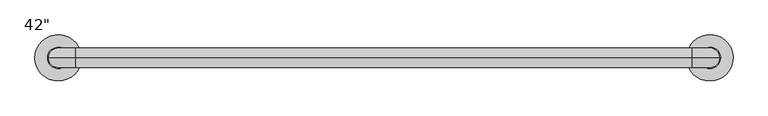
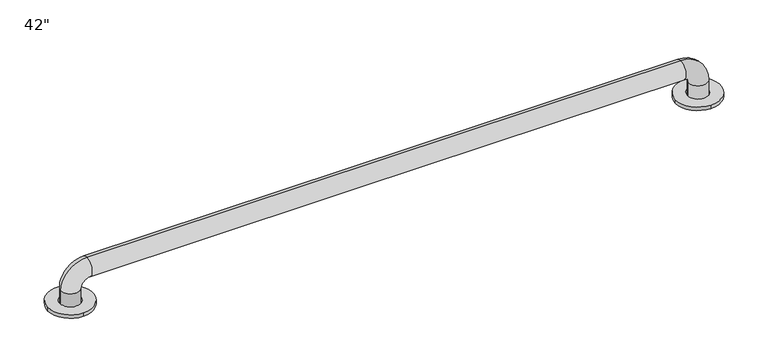
"""IFC4 building model written with IfcOpenShell, lengths in millimetres: proxy geometry."""

from ifc_helpers import new_model, si_unit, point, frame, frame_2d, origin, origin_with_axes, origin_2d, place, context, project, spatial, circle_curve, ellipse_curve, trimmed, segment, composite_curve, outline, extrude, source, transform, mapped, element, save
from ifc_brep_helpers import plane_surface, cylinder_surface, revolved_surface, advanced_brep


def proxy_a4e7295d(model_context):
    return source(origin(), model_context, "Body", "SolidModel", [
        extrude(outline(composite_curve([segment(trimmed(circle_curve(frame_2d((1066.8, 0.0)), 38.1), [point((1028.7, 0.0))], [point((1066.8, -38.1))], False, "CARTESIAN"), True, "CONTINUOUS"), segment(trimmed(circle_curve(frame_2d((1066.8, 0.0)), 38.1), [point((1066.8, -38.1))], [point((1028.7, 0.0))], False, "CARTESIAN"), True, "CONTINUOUS")], self_intersect=False), holes=[composite_curve([segment(trimmed(circle_curve(frame_2d((1066.8, 0.0)), 17.4625), [point((1049.3375, 0.0))], [point((1066.8, -17.4625))], True, "CARTESIAN"), True, "CONTINUOUS"), segment(trimmed(circle_curve(frame_2d((1066.8, 0.0)), 17.4625), [point((1066.8, -17.4625))], [point((1049.3375, 0.0))], True, "CARTESIAN"), True, "CONTINUOUS")], self_intersect=False)]), origin_with_axes(), (0.0, 0.0, 1.0), 6.35),
        extrude(outline(composite_curve([segment(trimmed(circle_curve(origin_2d(), 38.1), [point((-38.1, 0.0))], [point((0.0, -38.1))], False, "CARTESIAN"), True, "CONTINUOUS"), segment(trimmed(circle_curve(origin_2d(), 38.1), [point((0.0, -38.1))], [point((-38.1, 0.0))], False, "CARTESIAN"), True, "CONTINUOUS")], self_intersect=False), holes=[composite_curve([segment(trimmed(circle_curve(origin_2d(), 17.4625), [point((-17.4625, 0.0))], [point((0.0, -17.4625))], True, "CARTESIAN"), True, "CONTINUOUS"), segment(trimmed(circle_curve(origin_2d(), 17.4625), [point((0.0, -17.4625))], [point((-17.4625, 0.0))], True, "CARTESIAN"), True, "CONTINUOUS")], self_intersect=False)]), origin_with_axes(), (0.0, 0.0, 1.0), 6.35),
        advanced_brep(
        [(1082.675, 0.0, 0.0), (1050.925, 0.0, 0.0), (1082.675, 0.0, 28.575), (1050.925, 0.0, 28.575), (1038.225, 0.0, 41.275), (1038.225, 0.0, 73.025), (28.575, 0.0, 73.025), (28.575, 0.0, 41.275), (15.875, 0.0, 28.575), (-15.875, 0.0, 28.575), (-15.875, 0.0, 0.0), (15.875, 0.0, 0.0)],
        [
            (0, 1, circle_curve(frame((1066.8, 0.0, 0.0), z_axis=(0.0, 0.0, -1.0), x_axis=(-1.0, 0.0, 0.0)), 15.875)),
            (1, 0, circle_curve(frame((1066.8, 0.0, 0.0), z_axis=(0.0, 0.0, -1.0), x_axis=(-1.0, 0.0, 0.0)), 15.875)),
            (0, 2),
            (2, 3, circle_curve(frame((1066.8, 0.0, 28.575), z_axis=(0.0, 0.0, -1.0), x_axis=(-1.0, 0.0, 0.0)), 15.875)),
            (3, 1),
            (3, 2, circle_curve(frame((1066.8, 0.0, 28.575), z_axis=(0.0, 0.0, -1.0), x_axis=(-1.0, 0.0, 0.0)), 15.875)),
            (4, 3, circle_curve(frame((1038.225, 0.0, 28.575), z_axis=(0.0, 1.0, 0.0), x_axis=(1.0, 0.0, 0.0)), 12.7)),
            (2, 5, circle_curve(frame((1038.225, 0.0, 28.575), z_axis=(0.0, -1.0, 0.0), x_axis=(1.0, 0.0, 0.0)), 44.45)),
            (5, 4, circle_curve(frame((1038.225, 0.0, 57.15), z_axis=(1.0, 0.0, 0.0), x_axis=(0.0, 0.0, -1.0)), 15.875)),
            (4, 5, circle_curve(frame((1038.225, 0.0, 57.15), z_axis=(1.0, 0.0, 0.0), x_axis=(0.0, 0.0, -1.0)), 15.875)),
            (5, 6),
            (6, 7, circle_curve(frame((28.575, 0.0, 57.15), z_axis=(1.0, 0.0, 0.0), x_axis=(0.0, 0.0, -1.0)), 15.875)),
            (7, 4),
            (7, 6, circle_curve(frame((28.575, 0.0, 57.15), z_axis=(1.0, 0.0, 0.0), x_axis=(0.0, 0.0, -1.0)), 15.875)),
            (8, 7, circle_curve(frame((28.575, 0.0, 28.575), z_axis=(0.0, 1.0, 0.0), x_axis=(0.0, 0.0, 1.0)), 12.7)),
            (6, 9, circle_curve(frame((28.575, 0.0, 28.575), z_axis=(0.0, -1.0, 0.0), x_axis=(0.0, 0.0, 1.0)), 44.45)),
            (9, 8, circle_curve(frame((0.0, 0.0, 28.575), z_axis=(0.0, 0.0, 1.0), x_axis=(1.0, 0.0, 0.0)), 15.875)),
            (8, 9, circle_curve(frame((0.0, 0.0, 28.575), z_axis=(0.0, 0.0, 1.0), x_axis=(1.0, 0.0, 0.0)), 15.875)),
            (10, 11, circle_curve(frame((0.0, 0.0, 0.0), z_axis=(0.0, 0.0, -1.0), x_axis=(1.0, 0.0, 0.0)), 15.875)),
            (11, 10, circle_curve(frame((0.0, 0.0, 0.0), z_axis=(0.0, 0.0, -1.0), x_axis=(1.0, 0.0, 0.0)), 15.875)),
            (9, 10),
            (11, 8),
        ],
        [
            plane_surface(frame((1066.8, 0.0, 0.0), z_axis=(0.0, 0.0, -1.0), x_axis=(0.0, -1.0, 0.0))),
            cylinder_surface(frame((1066.8, 0.0, 0.0), z_axis=(0.0, 0.0, -1.0), x_axis=(-1.0, 0.0, 0.0)), 15.875),
            revolved_surface(trimmed(ellipse_curve(frame((1066.8, 0.0, 28.575), z_axis=(0.0, 0.0, -1.0), x_axis=(-1.0, 0.0, 0.0)), 15.875, 15.875), [point((1082.675, 0.0, 28.575))], [point((1050.925, 0.0, 28.575))], True, "CARTESIAN"), (1038.225, 0.0, 28.575), (0.0, -1.0, 0.0)),
            revolved_surface(trimmed(ellipse_curve(frame((1066.8, 0.0, 28.575), z_axis=(0.0, 0.0, -1.0), x_axis=(-1.0, 0.0, 0.0)), 15.875, 15.875), [point((1050.925, 0.0, 28.575))], [point((1082.675, 0.0, 28.575))], True, "CARTESIAN"), (1038.225, 0.0, 28.575), (0.0, -1.0, 0.0)),
            cylinder_surface(frame((1038.225, 0.0, 57.15), z_axis=(1.0, 0.0, 0.0), x_axis=(0.0, 0.0, -1.0)), 15.875),
            revolved_surface(trimmed(ellipse_curve(frame((28.575, 0.0, 57.15), z_axis=(1.0, 0.0, 0.0), x_axis=(0.0, 0.0, -1.0)), 15.875, 15.875), [point((28.575, 0.0, 73.025))], [point((28.575, 0.0, 41.275))], True, "CARTESIAN"), (28.575, 0.0, 28.575), (0.0, -1.0, 0.0)),
            revolved_surface(trimmed(ellipse_curve(frame((28.575, 0.0, 57.15), z_axis=(1.0, 0.0, 0.0), x_axis=(0.0, 0.0, -1.0)), 15.875, 15.875), [point((28.575, 0.0, 41.275))], [point((28.575, 0.0, 73.025))], True, "CARTESIAN"), (28.575, 0.0, 28.575), (0.0, -1.0, 0.0)),
            plane_surface(frame((0.0, 0.0, 0.0), z_axis=(0.0, 0.0, -1.0), x_axis=(0.0, -1.0, 0.0))),
            cylinder_surface(frame((0.0, 0.0, 28.575), z_axis=(0.0, 0.0, 1.0), x_axis=(1.0, 0.0, 0.0)), 15.875),
        ],
        [
            (0, [[1, 2]]),
            (1, [[-1, 3, 4, 5]]),
            (1, [[-2, -5, 6, -3]]),
            (2, [[7, -4, 8, 9]]),
            (3, [[-8, -6, -7, 10]]),
            (4, [[-9, 11, 12, 13]]),
            (4, [[-10, -13, 14, -11]]),
            (5, [[15, -12, 16, 17]]),
            (6, [[-16, -14, -15, 18]]),
            (7, [[19, 20]]),
            (8, [[-17, 21, -20, 22]]),
            (8, [[-18, -22, -19, -21]]),
        ],
    ),
    ])


if __name__ == "__main__":
    model = new_model("IFC4")
    model_context = context("Model", 3, world=origin())
    ifc_project = project(units=[si_unit("LENGTHUNIT", "METRE", prefix="MILLI")], contexts=[model_context])
    site = spatial("IfcSite", under=ifc_project)
    building = spatial("IfcBuilding", under=site)
    placement = place(None, origin())
    proxy_shape = proxy_a4e7295d(model_context)
    element("IfcBuildingElementProxy", 1, Name="Seqm-Grab Bar : 42\"", ObjectType="Seqm-Grab Bar : 42\"", at=placement, inside=building, context=model_context, shape_type="MappedRepresentation", body=[
        mapped(proxy_shape, transform((0.0, 0.0, 0.0), x_axis=(1.0, 0.0, 0.0), y_axis=(0.0, 1.0, 0.0), z_axis=(0.0, 0.0, 1.0))),
    ])
    save(model, "model.ifc")

# Revit data of these elements
# Type "Seqm-Grab Bar : 42\""
#   Spec Number = "10 28 00"
#   Spec Description = "42\" GRAB BAR"
#   Length = 3' - 6"
#   Default Elevation = 4' - 0"
#   Grab Bar Material = GRAB BARS - AT ADA RESTROOMS ONLY
# Element 1 (IfcBuildingElementProxy, "Seqm-Grab Bar : 42\"")
#   Materials on its faces: "GRAB BARS - AT ADA RESTROOMS ONLY"
# Materials
#   "GRAB BARS - AT ADA RESTROOMS ONLY": class "Generic", colour RGB 120 120 120, transparency 0, Cost = 0
